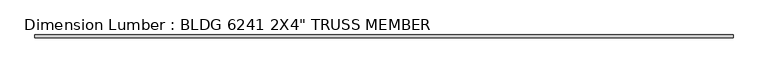
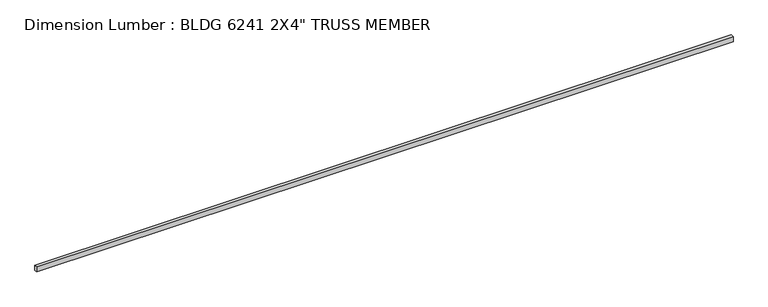
"""IFC4 building model written with IfcOpenShell, lengths in millimetres: beam geometry."""

from ifc_helpers import new_model, si_unit, frame, origin, place, context, project, spatial, polyline, outline, extrude, source, transform, mapped, element, save


def beam_5a8d2df6(model_context):
    return source(origin(), model_context, "Body", "SweptSolid", [
        extrude(outline(polyline([(6349.9999994, 25.4), (6349.9999994, -25.4), (-6288.6789755, -25.4), (-6288.6789755, 25.4), (6349.9999994, 25.4)])), frame((0.0, 0.0, -50.8), z_axis=(0.0, 0.0, 1.0), x_axis=(1.0, 0.0, 0.0)), (0.0, 0.0, 1.0), 101.6),
    ])


if __name__ == "__main__":
    model = new_model("IFC4")
    model_context = context("Model", 3, world=origin())
    ifc_project = project(units=[si_unit("LENGTHUNIT", "METRE", prefix="MILLI")], contexts=[model_context])
    site = spatial("IfcSite", under=ifc_project)
    building = spatial("IfcBuilding", under=site)
    placement = place(None, origin())
    beam_shape = beam_5a8d2df6(model_context)
    element("IfcBeam", 1, ObjectType="Dimension Lumber : BLDG 6241 2X4\" TRUSS MEMBER", at=placement, inside=building, context=model_context, shape_type="MappedRepresentation", body=[
        mapped(beam_shape, transform((0.0, 0.0, 0.0), x_axis=(1.0, 0.0, 0.0), y_axis=(0.0, 1.0, 0.0), z_axis=(0.0, 0.0, 1.0))),
    ])
    save(model, "model.ifc")

# Revit data of these elements
# Type "Dimension Lumber : BLDG 6241 2X4\" TRUSS MEMBER"
#   Assembly Code = "B10"
#   A = 0.273472 SF
#   Length [instance default] = 5' - 0"
#   b = 0' - 2"
#   d = 0' - 4"
#   Structural Material [instance default] = Softwood, Lumber
# Element 1 (IfcBeam, "Dimension Lumber : BLDG 6241 2X4\" TRUSS MEMBER")
#   Materials on its faces: "Softwood, Lumber"
# Materials
#   "Softwood, Lumber": class "Wood", colour RGB 223 192 134, transparency 0, Description = "Pinus Echinata", Cost = 0
